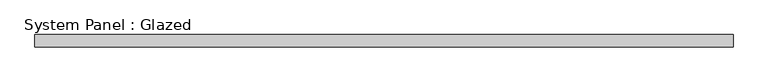
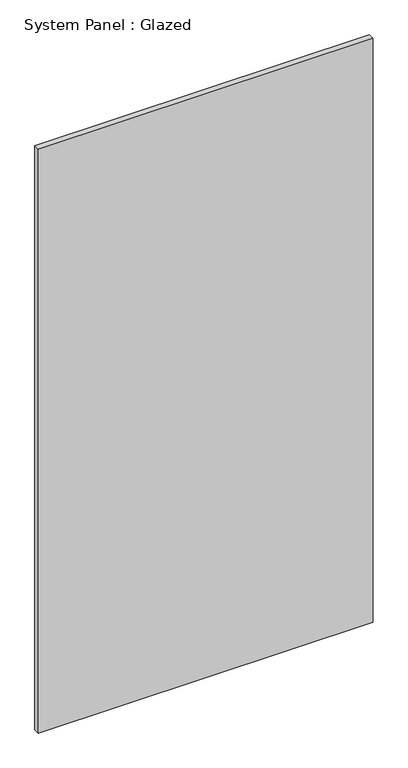
"""IFC4 building model written with IfcOpenShell, lengths in millimetres: plate geometry, System Panel : Glazed."""

from ifc_helpers import new_model, si_unit, origin, origin_with_axes, place, context, project, spatial, polyline, outline, extrude, source, transform, mapped, element, save


def system_panel_glazed_ef639d2b(model_context):
    return source(origin(), model_context, "Body", "SweptSolid", [
        extrude(outline(polyline([(712.5000001, 24.5), (-712.5000001, 24.5), (-712.5000001, 49.5), (712.5000001, 49.5), (712.5000001, 24.5)])), origin_with_axes(), (0.0, 0.0, 1.0), 2625.0),
    ])


if __name__ == "__main__":
    model = new_model("IFC4")
    model_context = context("Model", 3, world=origin())
    ifc_project = project(units=[si_unit("LENGTHUNIT", "METRE", prefix="MILLI")], contexts=[model_context])
    site = spatial("IfcSite", under=ifc_project)
    building = spatial("IfcBuilding", under=site)
    placement = place(None, origin())
    system_panel_glazed_shape = system_panel_glazed_ef639d2b(model_context)
    element("IfcPlate", 1, ObjectType="System Panel : Glazed", at=placement, inside=building, context=model_context, shape_type="MappedRepresentation", body=[
        mapped(system_panel_glazed_shape, transform((0.0, 0.0, 0.0), x_axis=(1.0, 0.0, 0.0), y_axis=(0.0, 1.0, 0.0), z_axis=(0.0, 0.0, 1.0))),
    ])
    save(model, "model.ifc")

# Revit data of these elements
# Type "System Panel : Glazed"
#   Keynote = "H11"
#   Construction Type Id = "GSP4R"
#   Analytic Construction = "1/8 in Pilkington single glazing"
#   Visual Light Transmittance = 0.9
#   Solar Heat Gain Coefficient = 0.86
#   Heat Transfer Coefficient (U) = 6.7069 W/(m²·K)
# Element 1 (IfcPlate, "System Panel : Glazed")
#   Materials on its faces: "Glass"
# Materials
#   "Glass": class "Glass", colour RGB 0 128 192, transparency 0.9, Description = "Soda Lime Glass", Cost = 0
